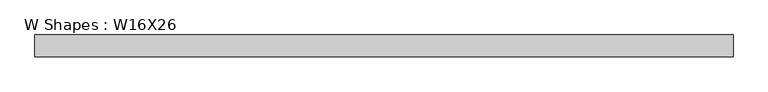
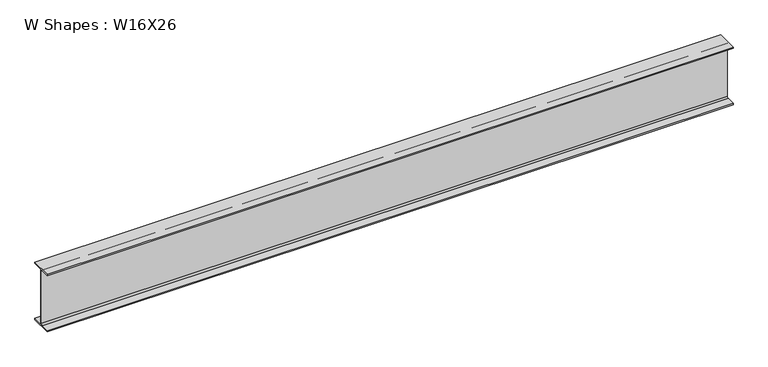
"""IFC4 building model written with IfcOpenShell, lengths in millimetres: beam geometry, W Shapes : W16X26."""

from ifc_helpers import new_model, si_unit, point, frame, frame_2d, origin, place, context, project, spatial, polyline, circle_curve, trimmed, segment, composite_curve, outline, extrude, source, transform, mapped, element, save


def w_shapes_w16x26_d059226d(model_context):
    return source(origin(), model_context, "Body", "SweptSolid", [
        extrude(outline(composite_curve([segment(polyline([(69.85, -190.627), (69.85, -199.39), (-69.85, -199.39), (-69.85, -190.627), (-13.3858, -190.627)]), True, "CONTINUOUS"), segment(trimmed(circle_curve(frame_2d((-13.3858, -180.4162)), 10.2108), [point((-13.3858, -190.627))], [point((-3.175, -180.4162))], True, "CARTESIAN"), True, "CONTINUOUS"), segment(polyline([(-3.175, -180.4162), (-3.175, 180.4162)]), True, "CONTINUOUS"), segment(trimmed(circle_curve(frame_2d((-13.3858, 180.4162)), 10.2108), [point((-3.175, 180.4162))], [point((-13.3858, 190.627))], True, "CARTESIAN"), True, "CONTINUOUS"), segment(polyline([(-13.3858, 190.627), (-69.85, 190.627), (-69.85, 199.39), (69.85, 199.39), (69.85, 190.627), (13.3858, 190.627)]), True, "CONTINUOUS"), segment(trimmed(circle_curve(frame_2d((13.3858, 180.4162)), 10.2108), [point((13.3858, 190.627))], [point((3.175, 180.4162))], True, "CARTESIAN"), True, "CONTINUOUS"), segment(polyline([(3.175, 180.4162), (3.175, -180.4162)]), True, "CONTINUOUS"), segment(trimmed(circle_curve(frame_2d((13.3858, -180.4162)), 10.2108), [point((3.175, -180.4162))], [point((13.3858, -190.627))], True, "CARTESIAN"), True, "CONTINUOUS"), segment(polyline([(13.3858, -190.627), (69.85, -190.627)]), True, "CONTINUOUS")], self_intersect=False)), frame((-2247.9, 0.0, 0.0), z_axis=(1.0, 0.0, 0.0), x_axis=(0.0, 1.0, 0.0)), (0.0, 0.0, 1.0), 4495.8),
    ])


if __name__ == "__main__":
    model = new_model("IFC4")
    model_context = context("Model", 3, world=origin())
    ifc_project = project(units=[si_unit("LENGTHUNIT", "METRE", prefix="MILLI")], contexts=[model_context])
    site = spatial("IfcSite", under=ifc_project)
    building = spatial("IfcBuilding", under=site)
    placement = place(None, origin())
    w_shapes_w16x26_shape = w_shapes_w16x26_d059226d(model_context)
    element("IfcBeam", 1, ObjectType="W Shapes : W16X26", at=placement, inside=building, context=model_context, shape_type="MappedRepresentation", body=[
        mapped(w_shapes_w16x26_shape, transform((0.0, 0.0, 0.0), x_axis=(1.0, 0.0, 0.0), y_axis=(0.0, 1.0, 0.0), z_axis=(0.0, 0.0, 1.0))),
    ])
    save(model, "model.ifc")

# Revit data of these elements
# Type "W Shapes : W16X26"
#   Section Name Key = "W16x26"
#   Assembly Code = "B10"
#   Width = 5.500"
#   Web Thickness = 0.250"
#   Web Fillet = 0.402"
#   Warping Constant = 565.00 in⁶
#   Torsional Moment of Inertia = 0.262 in⁴
#   Section Area = 7.68 in²
#   Plastic Modulus weak axis = 5.48 in³
#   Plastic Modulus strong axis = 44.20 in³
#   Perimeter = 4.35 ft²/ft
#   Nominal Weight = 26.00 lbf/ft
#   Moment of Inertia weak axis = 9.59 in⁴
#   Moment of Inertia strong axis = 301.00 in⁴
#   Height = 15.700"
#   Flange Thickness = 0.345"
#   Elastic Modulus weak axis = 3.49 in³
#   Elastic Modulus strong axis = 38.40 in³
#   Centroid Vertical = 7.850"
#   Centroid Horizontal = 2.750"
#   Bolt Spacing = 0' - 3 1/2"
#   Length [instance default] = 5' - 0"
#   Structural Material [instance default] = Steel ASTM A992
#   Principal Axes Angle = 0
# Element 1 (IfcBeam, "W Shapes : W16X26")
#   Structural Material = Steel ASTM A36
#   Materials on its faces: "Steel ASTM A36"
# Materials
#   "Steel ASTM A992": class "Metal", colour RGB 199 199 199, transparency 0, Description = "Structural steel 50ksi", Cost = 0
#   "Steel ASTM A36": class "Metal", colour RGB 199 199 199, transparency 0, Description = "Structural steel, ASTM A36 Grade B, mill finish", Cost = 0
